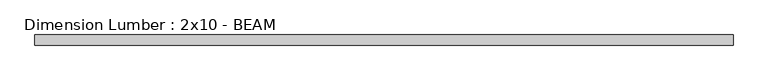
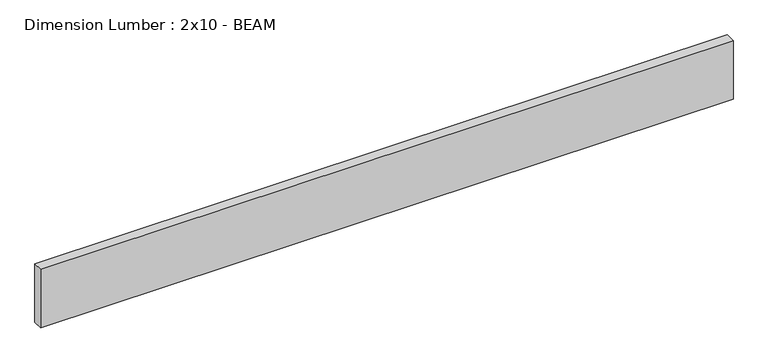
"""IFC4 building model written with IfcOpenShell, lengths in millimetres: beam geometry, Dimension Lumber : 2x10 - BEAM."""

from ifc_helpers import new_model, si_unit, frame, origin, place, context, project, spatial, polyline, outline, extrude, source, transform, mapped, element, save


def dimension_lumber_2x10_beam_d8784499(model_context):
    return source(origin(), model_context, "Body", "SweptSolid", [
        extrude(outline(polyline([(1315.9630859, 19.05), (1315.9630859, -19.05), (-1315.9630859, -19.05), (-1315.9630859, 19.05), (1315.9630859, 19.05)])), frame((0.0, 0.0, -117.475), z_axis=(0.0, 0.0, 1.0), x_axis=(1.0, 0.0, 0.0)), (0.0, 0.0, 1.0), 234.95),
    ])


if __name__ == "__main__":
    model = new_model("IFC4")
    model_context = context("Model", 3, world=origin())
    ifc_project = project(units=[si_unit("LENGTHUNIT", "METRE", prefix="MILLI")], contexts=[model_context])
    site = spatial("IfcSite", under=ifc_project)
    building = spatial("IfcBuilding", under=site)
    placement = place(None, origin())
    dimension_lumber_2x10_beam_shape = dimension_lumber_2x10_beam_d8784499(model_context)
    element("IfcBeam", 1, ObjectType="Dimension Lumber : 2x10 - BEAM", at=placement, inside=building, context=model_context, shape_type="MappedRepresentation", body=[
        mapped(dimension_lumber_2x10_beam_shape, transform((0.0, 0.0, 0.0), x_axis=(1.0, 0.0, 0.0), y_axis=(0.0, 1.0, 0.0), z_axis=(0.0, 0.0, 1.0))),
    ])
    save(model, "model.ifc")

# Revit data of these elements
# Type "Dimension Lumber : 2x10 - BEAM"
#   Assembly Code = "B10"
#   A = 0.0755556 SF
#   Length [instance default] = 5' - 0"
#   b = 0' - 1 1/2"
#   d = 0' - 9 1/4"
#   Structural Material = (3) SISTERED 2X10s AT BEAM
# Element 1 (IfcBeam, "Dimension Lumber : 2x10 - BEAM")
#   Materials on its faces: "(3) SISTERED 2X10s AT BEAM"
# Materials
#   "(3) SISTERED 2X10s AT BEAM": class "Wood", colour RGB 234 198 147, transparency 0, Description = "Pinus Echinata", Cost = 0
